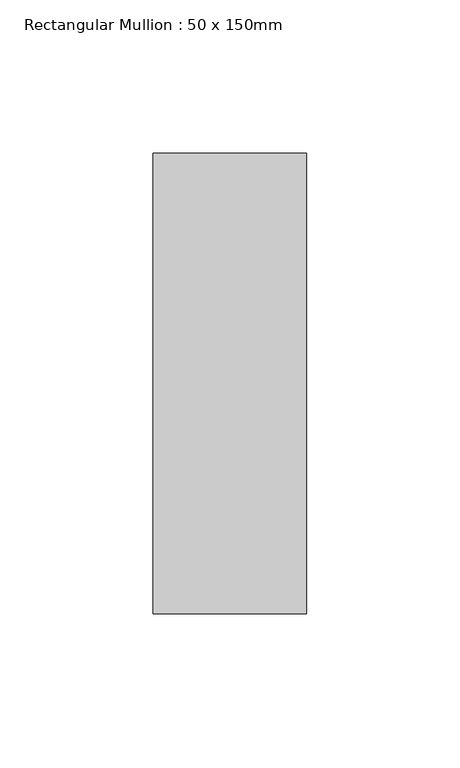
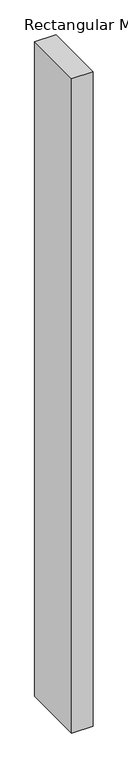
"""IFC4 building model written with IfcOpenShell, lengths in millimetres: member geometry, Rectangular Mullion : 50 x 150mm."""

import ifcopenshell
import ifcopenshell.guid

model = None  # the IFC model being written
_history = None  # IfcOwnerHistory: only IFC2X3 demands one
_inside = {}  # id of a spatial element -> (the spatial element, [elements in it])
_under = {}  # id of a project, library or spatial element -> (it, [spatial elements below it])
_declared = {}  # id of a project -> (the project, [libraries it declares])
_typed = {}  # id of a type object -> (the type object, [elements of that type])
_made_of = {}  # id of a material, layer set ... -> (it, [elements and type objects made of it])


def new_model(schema):
    """Start an empty IFC model of exactly this schema.

    Asked for "IFC4X3", IfcOpenShell would pick the latest addendum, in which some entities
    have other attributes; the version numbers below select the first issue.
    IFC2X3 requires an IfcOwnerHistory on every rooted entity: one is made here for all.
    """
    global model, _history
    if schema == "IFC4X3":
        model = ifcopenshell.file(schema_version=(4, 3, 0, 0))
    else:
        model = ifcopenshell.file(schema=schema)
    _inside.clear()
    _under.clear()
    _declared.clear()
    _typed.clear()
    _made_of.clear()
    _history = None
    if model.schema == "IFC2X3":
        org = make("IfcOrganization", Name="unknown")
        user = make(
            "IfcPersonAndOrganization",
            ThePerson=make("IfcPerson", FamilyName="unknown"),
            TheOrganization=org,
        )
        app = make(
            "IfcApplication",
            ApplicationDeveloper=org,
            Version="unknown",
            ApplicationFullName="unknown",
            ApplicationIdentifier="unknown",
        )
        _history = make(
            "IfcOwnerHistory",
            OwningUser=user,
            OwningApplication=app,
            ChangeAction="ADDED",
            CreationDate=0,
        )
    return model


def make(cls, **values):
    """One entity of the class cls with the attributes given. An attribute that is None is left unset."""
    return model.create_entity(
        cls, **{name: value for name, value in values.items() if value is not None}
    )


def rooted(cls, **values):
    """An entity with a GlobalId (a new one), such as an element, a storey or a relation."""
    return make(cls, GlobalId=ifcopenshell.guid.new(), OwnerHistory=_history, **values)


def si_unit(unit_type, name, prefix=None):
    """IfcSIUnit, for example si_unit("LENGTHUNIT", "METRE", prefix="MILLI")."""
    return make("IfcSIUnit", UnitType=unit_type, Prefix=prefix, Name=name)


def assignment(units):
    """IfcUnitAssignment: the units of a project."""
    return None if units is None else make("IfcUnitAssignment", Units=units)


def point(xyz):
    """IfcCartesianPoint."""
    return None if xyz is None else make("IfcCartesianPoint", Coordinates=xyz)


def direction(xyz):
    """IfcDirection."""
    return None if xyz is None else make("IfcDirection", DirectionRatios=xyz)


def frame(location, z_axis=None, x_axis=None):
    """IfcAxis2Placement3D, a coordinate frame: its origin and axes. An axis left out is left unset."""
    return make(
        "IfcAxis2Placement3D",
        Location=point(location),
        Axis=direction(z_axis),
        RefDirection=direction(x_axis),
    )


def origin():
    """The frame at (0, 0, 0) with its axes left unset."""
    return frame((0.0, 0.0, 0.0))


def place(relative_to, where):
    """IfcLocalPlacement: puts the frame where relative to a parent placement (None: the world)."""
    return make(
        "IfcLocalPlacement", PlacementRelTo=relative_to, RelativePlacement=where
    )


def context(
    kind, dimensions, precision=None, world=None, true_north=None, identifier=None
):
    """IfcGeometricRepresentationContext, for example the 3D "Model" context."""
    return make(
        "IfcGeometricRepresentationContext",
        ContextIdentifier=identifier,
        ContextType=kind,
        CoordinateSpaceDimension=dimensions,
        Precision=precision,
        WorldCoordinateSystem=world,
        TrueNorth=true_north,
    )


def project(units=None, contexts=None):
    """IfcProject with its units and contexts."""
    return rooted(
        "IfcProject",
        Name="project",
        RepresentationContexts=contexts,
        UnitsInContext=assignment(units),
    )


def spatial(cls, under=None, at=None, **own):
    """A site, building, storey or space (cls), placed at a placement, below another one or the project."""
    s = rooted(cls, ObjectPlacement=at, **own)
    if under is not None:
        _under.setdefault(under.id(), (under, []))[1].append(s)
    return s


def polyline(points):
    """IfcPolyline through the points."""
    return make("IfcPolyline", Points=[point(p) for p in points])


def outline(outer, holes=None, kind="AREA"):
    """IfcArbitraryClosedProfileDef: a profile drawn as a closed curve; with holes, ...WithVoids."""
    if holes is None:
        return make("IfcArbitraryClosedProfileDef", ProfileType=kind, OuterCurve=outer)
    return make(
        "IfcArbitraryProfileDefWithVoids",
        ProfileType=kind,
        OuterCurve=outer,
        InnerCurves=holes,
    )


def extrude(swept, where, along, depth):
    """IfcExtrudedAreaSolid: the profile swept, set in the frame where, extruded along a direction by depth."""
    return make(
        "IfcExtrudedAreaSolid",
        SweptArea=swept,
        Position=where,
        ExtrudedDirection=direction(along),
        Depth=depth,
    )


def shape(context_of_items, identifier, shape_type, items):
    """IfcShapeRepresentation: the items that make up one representation, for example the "Body"."""
    return make(
        "IfcShapeRepresentation",
        ContextOfItems=context_of_items,
        RepresentationIdentifier=identifier,
        RepresentationType=shape_type,
        Items=items,
    )


def source(mapping_origin, context_of_items, identifier, shape_type, items):
    """IfcRepresentationMap: a shape defined once, which mapped items show again and again."""
    return make(
        "IfcRepresentationMap",
        MappingOrigin=mapping_origin,
        MappedRepresentation=shape(context_of_items, identifier, shape_type, items),
    )


def transform(
    local_origin,
    x_axis=None,
    y_axis=None,
    z_axis=None,
    scale=None,
    scale2=None,
    scale3=None,
    uniform=True,
):
    """IfcCartesianTransformationOperator3D, or its non-uniform kind. x_axis, y_axis, z_axis: its Axis1, 2, 3."""
    if uniform:
        return make(
            "IfcCartesianTransformationOperator3D",
            Axis1=direction(x_axis),
            Axis2=direction(y_axis),
            LocalOrigin=point(local_origin),
            Scale=scale,
            Axis3=direction(z_axis),
        )
    return make(
        "IfcCartesianTransformationOperator3DnonUniform",
        Axis1=direction(x_axis),
        Axis2=direction(y_axis),
        LocalOrigin=point(local_origin),
        Scale=scale,
        Axis3=direction(z_axis),
        Scale2=scale2,
        Scale3=scale3,
    )


def mapped(mapping_source, mapping_target):
    """IfcMappedItem: shows the shape of a source again, moved by a transform."""
    return make(
        "IfcMappedItem", MappingSource=mapping_source, MappingTarget=mapping_target
    )


def made_of(thing, what):
    """Note that an element or type object is made of a material, layer set ...; save() writes the relation."""
    if what is not None:
        _made_of.setdefault(what.id(), (what, []))[1].append(thing)
    return thing


def element(
    cls,
    number,
    at=None,
    inside=None,
    cuts=None,
    type_object=None,
    material=None,
    context=None,
    identifier="Body",
    shape_type=None,
    held_by="IfcProductDefinitionShape",
    body=None,
    shapes=None,
    **own,
):
    """One element of the class cls, such as IfcWall. Its Tag is "e" and its number.

    at: its placement. inside: the storey or other place that contains it. cuts: it is an
    opening in that element (IfcRelVoidsElement). A single representation is given by context,
    identifier, shape_type and body (its items); several are given by shapes. held_by: the class
    of the entity that holds the representations. save() writes the other relations.
    """
    e = rooted(cls, Tag="e%d" % number, ObjectPlacement=at, **own)
    if body is not None:
        shapes = [shape(context, identifier, shape_type, body)]
    if shapes is not None:
        e.Representation = make(held_by, Representations=shapes)
    if inside is not None:
        _inside.setdefault(inside.id(), (inside, []))[1].append(e)
    if cuts is not None:
        rooted(
            "IfcRelVoidsElement", RelatingBuildingElement=cuts, RelatedOpeningElement=e
        )
    if type_object is not None:
        _typed.setdefault(type_object.id(), (type_object, []))[1].append(e)
    return made_of(e, material)


def aggregate(whole, parts):
    """IfcRelAggregates: a whole, such as a stair, and the parts it consists of."""
    return rooted("IfcRelAggregates", RelatingObject=whole, RelatedObjects=parts)


def save(model, path):
    """Write the relations noted so far, then the file.

    IfcRelAggregates (storeys below a building ...), IfcRelContainedInSpatialStructure (elements
    in a storey), IfcRelDefinesByType, IfcRelAssociatesMaterial and IfcRelDeclares: one each for
    every whole, place, type object, material and project.
    """
    for whole, parts in _under.values():
        aggregate(whole, parts)
    for where, things in _inside.values():
        rooted(
            "IfcRelContainedInSpatialStructure",
            RelatedElements=things,
            RelatingStructure=where,
        )
    for kind, things in _typed.values():
        rooted("IfcRelDefinesByType", RelatedObjects=things, RelatingType=kind)
    for what, things in _made_of.values():
        rooted("IfcRelAssociatesMaterial", RelatedObjects=things, RelatingMaterial=what)
    for by, libraries in _declared.values():
        rooted("IfcRelDeclares", RelatingContext=by, RelatedDefinitions=libraries)
    model.write(path)


def rectangular_mullion_50_x_150mm_a561114d(model_context):
    return source(origin(), model_context, "Body", "SweptSolid", [
        extrude(outline(polyline([(25.0, 75.0), (25.0, -75.0), (-25.0, -75.0), (-25.0, 75.0), (25.0, 75.0)])), frame((0.0, 0.0, -1615.55), z_axis=(0.0, 0.0, 1.0), x_axis=(1.0, 0.0, 0.0)), (0.0, 0.0, 1.0), 1615.55),
    ])


if __name__ == "__main__":
    model = new_model("IFC4")
    model_context = context("Model", 3, world=origin())
    ifc_project = project(units=[si_unit("LENGTHUNIT", "METRE", prefix="MILLI")], contexts=[model_context])
    site = spatial("IfcSite", under=ifc_project)
    building = spatial("IfcBuilding", under=site)
    placement = place(None, origin())
    rectangular_mullion_50_x_150mm_shape = rectangular_mullion_50_x_150mm_a561114d(model_context)
    element("IfcMember", 1, ObjectType="Rectangular Mullion : 50 x 150mm", at=placement, inside=building, context=model_context, shape_type="MappedRepresentation", body=[
        mapped(rectangular_mullion_50_x_150mm_shape, transform((0.0, 0.0, 0.0), x_axis=(1.0, 0.0, 0.0), y_axis=(0.0, 1.0, 0.0), z_axis=(0.0, 0.0, 1.0))),
    ])
    save(model, "model.ifc")

# Revit data of these elements
# Type "Rectangular Mullion : 50 x 150mm"
#   Keynote = "H11"
#   built-in parameter 1007304 = 0.492126 (stored number, unit not read)
#   built-in parameter 1007301 = 0.082021 (stored number, unit not read)
#   built-in parameter 1007300 = 0.082021 (stored number, unit not read)
# Element 1 (IfcMember, "Rectangular Mullion : 50 x 150mm")
#   Materials on its faces: "Aluminium"
# Materials
#   "Aluminium": class "Metal", colour RGB 247 247 247, transparency 0, Description = "Aluminium 6061", Cost = 0
